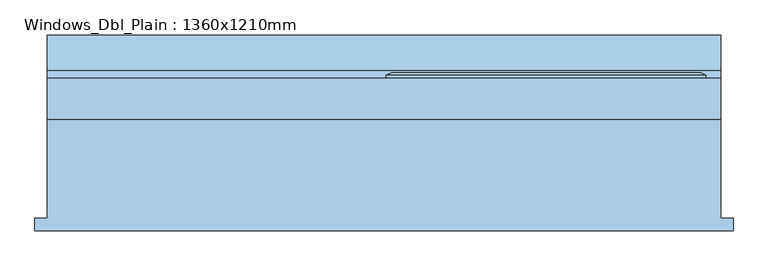
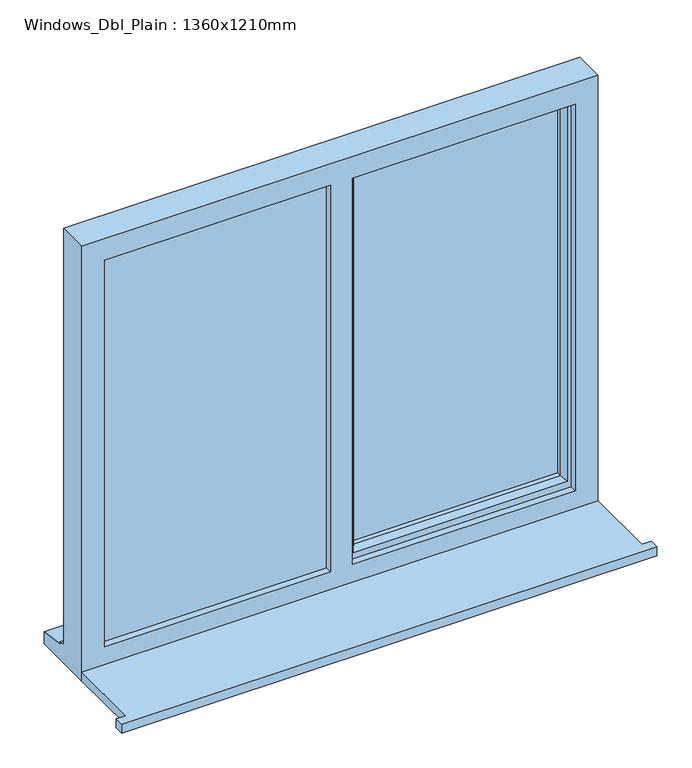
"""IFC4 building model written with IfcOpenShell, lengths in millimetres: window geometry, Windows_Dbl_Plain : 1360x1210mm."""

from ifc_helpers import new_model, si_unit, frame, origin, place, context, project, spatial, polyline, outline, extrude, faceted_brep, source, transform, mapped, element, save


def windows_dbl_plain_1360x1210mm_d7c3e583(model_context):
    return source(origin(), model_context, "Body", "SolidModel", [
        extrude(outline(polyline([(-990.0, -182.7934322), (-990.0, -157.7934322), (-965.0, -157.7934322), (-965.0, 41.7065678), (395.0, 41.7065678), (395.0, -157.7934322), (420.0, -157.7934322), (420.0, -182.7934322), (-990.0, -182.7934322)])), frame((0.0, 0.0, 900.0), z_axis=(0.0, 0.0, 1.0), x_axis=(1.0, 0.0, 0.0)), (0.0, 0.0, 1.0), 25.0),
        extrude(outline(polyline([(325.0, 88.7065678), (-240.0, 88.7065678), (-240.0, 112.7065678), (325.0, 112.7065678), (325.0, 88.7065678)])), frame((0.0, 0.0, 993.0), z_axis=(0.0, 0.0, 1.0), x_axis=(1.0, 0.0, 0.0)), (0.0, 0.0, 1.0), 1047.0),
        extrude(outline(polyline([(-925.0, 83.7065678), (-300.0, 83.7065678), (-300.0, 59.7065678), (-925.0, 59.7065678), (-925.0, 83.7065678)])), frame((0.0, 0.0, 963.0), z_axis=(0.0, 0.0, 1.0), x_axis=(1.0, 0.0, 0.0)), (0.0, 0.0, 1.0), 1107.0),
        faceted_brep([(395.0, 41.7065678, 2110.0), (-965.0, 41.7065678, 2110.0), (-965.0, 41.7065678, 900.0), (395.0, 41.7065678, 900.0), (335.0, 41.7065678, 2050.0), (335.0, 41.7065678, 975.0), (-252.0, 41.7065678, 975.0), (-252.0, 41.7065678, 2050.0), (-310.0, 41.7065678, 2050.0), (-310.0, 41.7065678, 975.0), (-905.0, 41.7065678, 975.0), (-905.0, 41.7065678, 2050.0), (-965.0, 124.7065678, 2110.0), (-965.0, 124.7065678, 951.0), (-965.0, 139.7065678, 949.68767), (-965.0, 139.7065678, 944.7449676), (-965.0, 212.2065678, 933.8088847), (-965.0, 212.2065678, 900.0), (395.0, 124.7065678, 2110.0), (395.0, 124.7065678, 951.0), (-925.0, 124.7065678, 2070.0), (-925.0, 124.7065678, 963.0), (-310.0, 124.7065678, 963.0), (-310.0, 124.7065678, 2070.0), (-270.0, 124.7065678, 2070.0), (-270.0, 124.7065678, 963.0), (355.0, 124.7065678, 963.0), (355.0, 124.7065678, 2070.0), (-925.0, 59.7065678, 2070.0), (-925.0, 59.7065678, 963.0), (-300.0, 59.7065678, 2070.0), (-300.0, 59.7065678, 963.0), (-310.0, 59.7065678, 2050.0), (-905.0, 59.7065678, 2050.0), (-905.0, 59.7065678, 975.0), (-310.0, 59.7065678, 975.0), (-270.0, 59.7065678, 2070.0), (355.0, 59.7065678, 2070.0), (355.0, 59.7065678, 963.0), (-270.0, 59.7065678, 963.0), (335.0, 59.7065678, 2050.0), (-252.0, 59.7065678, 2050.0), (-252.0, 59.7065678, 975.0), (335.0, 59.7065678, 975.0), (-310.0, 83.7065678, 2070.0), (-300.0, 83.7065678, 2070.0), (395.0, 212.2065678, 900.0), (395.0, 212.2065678, 933.8088847), (395.0, 139.7065678, 944.7449676), (395.0, 139.7065678, 949.68767), (-300.0, 83.7065678, 963.0), (-310.0, 83.7065678, 963.0)], [[[0, 1, 2, 3], [4, 5, 6, 7], [8, 9, 10, 11]], [[2, 1, 12, 13, 14, 15, 16, 17]], [[13, 12, 18, 19], [20, 21, 22, 23], [24, 25, 26, 27]], [[21, 20, 28, 29]], [[28, 30, 31, 29], [32, 33, 34, 35]], [[36, 37, 38, 39], [40, 41, 42, 43]], [[33, 11, 10, 34]], [[1, 0, 18, 12]], [[28, 20, 23, 44, 45, 30]], [[27, 37, 36, 24]], [[11, 33, 32, 8]], [[40, 4, 7, 41]], [[19, 18, 0, 3, 46, 47, 48, 49]], [[27, 26, 38, 37]], [[4, 40, 43, 5]], [[45, 50, 31, 30]], [[50, 45, 44, 51]], [[51, 44, 23, 22]], [[25, 24, 36, 39]], [[41, 7, 6, 42]], [[8, 32, 35, 9]], [[46, 3, 2, 17]], [[47, 46, 17, 16]], [[48, 47, 16, 15]], [[49, 48, 15, 14]], [[19, 49, 14, 13]], [[22, 21, 29, 31, 50, 51]], [[26, 25, 39, 38]], [[6, 5, 43, 42]], [[35, 34, 10, 9]]]),
        extrude(outline(polyline([(2050.0, -310.0), (2070.0, -310.0), (2070.0, -925.0), (963.0, -925.0), (963.0, -310.0), (983.0, -310.0), (983.0, -905.0), (2050.0, -905.0), (2050.0, -310.0)])), frame((0.0, 83.7065678, 0.0), z_axis=(0.0, 1.0, 0.0), x_axis=(0.0, 0.0, 1.0)), (0.0, 0.0, 1.0), 41.0),
        faceted_brep([(-280.0, 124.7065678, 2080.0), (-280.0, 130.4800705, 2080.0), (-280.0, 130.4800705, 953.0), (-280.0, 124.7065678, 953.0), (-270.0, 59.7065678, 2070.0), (-270.0, 124.7065678, 2070.0), (-270.0, 124.7065678, 963.0), (-270.0, 59.7065678, 963.0), (-230.0, 74.1994677, 2030.0), (-240.1480377, 59.7065678, 2040.1480377), (-240.1480377, 59.7065678, 992.8519623), (-230.0, 74.1994677, 1003.0), (-230.0, 88.7065678, 2030.0), (-230.0, 88.7065678, 1003.0), (-240.0, 112.7065678, 2040.0), (-240.0, 88.7065678, 2040.0), (-240.0, 88.7065678, 993.0), (-240.0, 112.7065678, 993.0), (-230.0, 130.4800705, 2030.0), (-230.0, 112.7065678, 2030.0), (-230.0, 112.7065678, 1003.0), (-230.0, 130.4800705, 1003.0), (-247.4457548, 136.2535732, 2047.4457548), (-247.4457548, 136.2535732, 985.5542452), (-269.2153903, 136.2535732, 2069.2153903), (-269.2153903, 136.2535732, 963.7846097), (365.0, 130.4800705, 953.0), (365.0, 124.7065678, 953.0), (355.0, 124.7065678, 963.0), (355.0, 59.7065678, 963.0), (325.1480377, 59.7065678, 992.8519623), (315.0, 74.1994677, 1003.0), (315.0, 88.7065678, 1003.0), (325.0, 88.7065678, 993.0), (325.0, 112.7065678, 993.0), (315.0, 112.7065678, 1003.0), (315.0, 130.4800705, 1003.0), (332.4457548, 136.2535732, 985.5542452), (354.2153903, 136.2535732, 963.7846097), (365.0, 130.4800705, 2080.0), (365.0, 124.7065678, 2080.0), (355.0, 124.7065678, 2070.0), (355.0, 59.7065678, 2070.0), (325.1480377, 59.7065678, 2040.1480377), (315.0, 74.1994677, 2030.0), (315.0, 88.7065678, 2030.0), (325.0, 88.7065678, 2040.0), (325.0, 112.7065678, 2040.0), (315.0, 112.7065678, 2030.0), (315.0, 130.4800705, 2030.0), (332.4457548, 136.2535732, 2047.4457548), (354.2153903, 136.2535732, 2069.2153903)], [[[0, 1, 2, 3]], [[4, 5, 6, 7]], [[8, 9, 10, 11]], [[12, 8, 11, 13]], [[14, 15, 16, 17]], [[18, 19, 20, 21]], [[22, 18, 21, 23]], [[1, 24, 25, 2]], [[3, 2, 26, 27]], [[7, 6, 28, 29]], [[11, 10, 30, 31]], [[13, 11, 31, 32]], [[17, 16, 33, 34]], [[21, 20, 35, 36]], [[23, 21, 36, 37]], [[2, 25, 38, 26]], [[27, 26, 39, 40]], [[29, 28, 41, 42]], [[31, 30, 43, 44]], [[32, 31, 44, 45]], [[34, 33, 46, 47]], [[36, 35, 48, 49]], [[37, 36, 49, 50]], [[26, 38, 51, 39]], [[40, 39, 1, 0]], [[3, 27, 40, 0], [5, 41, 28, 6]], [[42, 41, 5, 4]], [[7, 29, 42, 4], [9, 43, 30, 10]], [[44, 43, 9, 8]], [[45, 44, 8, 12]], [[15, 46, 33, 16], [13, 32, 45, 12]], [[47, 46, 15, 14]], [[17, 34, 47, 14], [19, 48, 35, 20]], [[49, 48, 19, 18]], [[50, 49, 18, 22]], [[24, 51, 38, 25], [23, 37, 50, 22]], [[39, 51, 24, 1]]]),
    ])


if __name__ == "__main__":
    model = new_model("IFC4")
    model_context = context("Model", 3, world=origin())
    ifc_project = project(units=[si_unit("LENGTHUNIT", "METRE", prefix="MILLI")], contexts=[model_context])
    site = spatial("IfcSite", under=ifc_project)
    building = spatial("IfcBuilding", under=site)
    placement = place(None, origin())
    windows_dbl_plain_1360x1210mm_shape = windows_dbl_plain_1360x1210mm_d7c3e583(model_context)
    element("IfcWindow", 1, ObjectType="Windows_Dbl_Plain : 1360x1210mm", at=placement, inside=building, context=model_context, shape_type="MappedRepresentation", body=[
        mapped(windows_dbl_plain_1360x1210mm_shape, transform((0.0, 0.0, 0.0), x_axis=(1.0, 0.0, 0.0), y_axis=(0.0, 1.0, 0.0), z_axis=(0.0, 0.0, 1.0))),
    ])
    save(model, "model.ifc")

# Revit data of these elements
# Type "Windows_Dbl_Plain : 1360x1210mm"
#   Type Mark = "83"
#   Operation = "DoublePanelVertical"
#   Construction Type Id = "GSP4R"
#   Manufacturer = "Revit"
#   Keynote = "L10"
#   Analytic Construction = "1/8 in Pilkington single glazing"
#   Wrap Layers (Ext) from Ext = 102.5 mm
#   Wrap Layers (Int) from Ext = 177.5 mm
#   Window Board Projection = 25 mm
#   Window Board Extension = 25 mm
#   Visual Light Transmittance = 0.9
#   Solar Heat Gain Coefficient = 0.78
#   Rough Width = 1360 mm
#   Rough Height = 1210 mm
#   Height = 1210 mm
#   Width = 1360 mm
#   Heat Transfer Coefficient (U) = 3.6886 W/(m²·K)
#   Glazing Thickness = 24 mm
#   FrameOffset - External = 50 mm
#   Frame Depth = 65 mm
#   Default Head Height = 2110 mm
#   Cill Depth = 87.5 mm
#   Cavity Closer Width = 50 mm
#   Cavity Closer Offset from Ext = 102.5 mm
#   Cavity Closer Depth = 85 mm
#   Vis - Cavity Closers = yes
#   Define Thermal Properties by = 1
#   Material Trim = Window Frame
#   Material Glass = Glass
#   Material Frame = Window Frame
#   Wall Closure = (empty or 0)
# Element 1 (IfcWindow, "Windows_Dbl_Plain : 1360x1210mm")
#   Materials on its faces: "Window Frame", "Glass"
# Materials
#   "Window Frame": class "Miscellaneous", colour RGB 249 249 249, transparency 0, Keynote = "L10"
#   "Glass": class "Glass", colour RGB 0 128 192, transparency 0.9, Description = "Soda Lime Glass", Cost = 0
